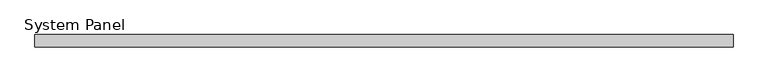
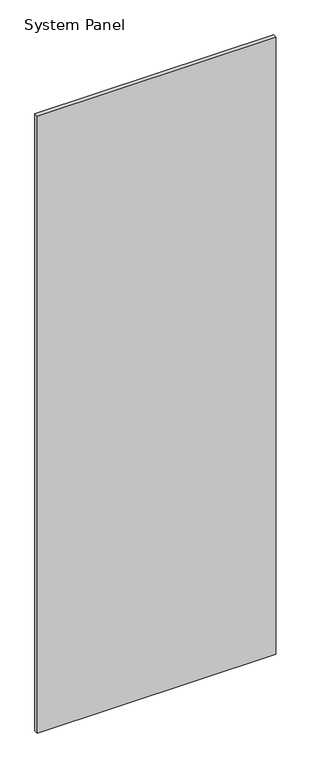
"""IFC4 building model written with IfcOpenShell, lengths in millimetres: plate geometry, System Panel : WWm-Glass-20mm-10mmOffset."""

import ifcopenshell
import ifcopenshell.guid

model = None  # the IFC model being written
_history = None  # IfcOwnerHistory: only IFC2X3 demands one
_inside = {}  # id of a spatial element -> (the spatial element, [elements in it])
_under = {}  # id of a project, library or spatial element -> (it, [spatial elements below it])
_declared = {}  # id of a project -> (the project, [libraries it declares])
_typed = {}  # id of a type object -> (the type object, [elements of that type])
_made_of = {}  # id of a material, layer set ... -> (it, [elements and type objects made of it])


def new_model(schema):
    """Start an empty IFC model of exactly this schema.

    Asked for "IFC4X3", IfcOpenShell would pick the latest addendum, in which some entities
    have other attributes; the version numbers below select the first issue.
    IFC2X3 requires an IfcOwnerHistory on every rooted entity: one is made here for all.
    """
    global model, _history
    if schema == "IFC4X3":
        model = ifcopenshell.file(schema_version=(4, 3, 0, 0))
    else:
        model = ifcopenshell.file(schema=schema)
    _inside.clear()
    _under.clear()
    _declared.clear()
    _typed.clear()
    _made_of.clear()
    _history = None
    if model.schema == "IFC2X3":
        org = make("IfcOrganization", Name="unknown")
        user = make(
            "IfcPersonAndOrganization",
            ThePerson=make("IfcPerson", FamilyName="unknown"),
            TheOrganization=org,
        )
        app = make(
            "IfcApplication",
            ApplicationDeveloper=org,
            Version="unknown",
            ApplicationFullName="unknown",
            ApplicationIdentifier="unknown",
        )
        _history = make(
            "IfcOwnerHistory",
            OwningUser=user,
            OwningApplication=app,
            ChangeAction="ADDED",
            CreationDate=0,
        )
    return model


def make(cls, **values):
    """One entity of the class cls with the attributes given. An attribute that is None is left unset."""
    return model.create_entity(
        cls, **{name: value for name, value in values.items() if value is not None}
    )


def rooted(cls, **values):
    """An entity with a GlobalId (a new one), such as an element, a storey or a relation."""
    return make(cls, GlobalId=ifcopenshell.guid.new(), OwnerHistory=_history, **values)


def si_unit(unit_type, name, prefix=None):
    """IfcSIUnit, for example si_unit("LENGTHUNIT", "METRE", prefix="MILLI")."""
    return make("IfcSIUnit", UnitType=unit_type, Prefix=prefix, Name=name)


def assignment(units):
    """IfcUnitAssignment: the units of a project."""
    return None if units is None else make("IfcUnitAssignment", Units=units)


def point(xyz):
    """IfcCartesianPoint."""
    return None if xyz is None else make("IfcCartesianPoint", Coordinates=xyz)


def direction(xyz):
    """IfcDirection."""
    return None if xyz is None else make("IfcDirection", DirectionRatios=xyz)


def frame(location, z_axis=None, x_axis=None):
    """IfcAxis2Placement3D, a coordinate frame: its origin and axes. An axis left out is left unset."""
    return make(
        "IfcAxis2Placement3D",
        Location=point(location),
        Axis=direction(z_axis),
        RefDirection=direction(x_axis),
    )


def origin():
    """The frame at (0, 0, 0) with its axes left unset."""
    return frame((0.0, 0.0, 0.0))


def origin_with_axes():
    """The frame at (0, 0, 0) with the z axis (0, 0, 1) and the x axis (1, 0, 0) written out."""
    return frame((0.0, 0.0, 0.0), z_axis=(0.0, 0.0, 1.0), x_axis=(1.0, 0.0, 0.0))


def place(relative_to, where):
    """IfcLocalPlacement: puts the frame where relative to a parent placement (None: the world)."""
    return make(
        "IfcLocalPlacement", PlacementRelTo=relative_to, RelativePlacement=where
    )


def context(
    kind, dimensions, precision=None, world=None, true_north=None, identifier=None
):
    """IfcGeometricRepresentationContext, for example the 3D "Model" context."""
    return make(
        "IfcGeometricRepresentationContext",
        ContextIdentifier=identifier,
        ContextType=kind,
        CoordinateSpaceDimension=dimensions,
        Precision=precision,
        WorldCoordinateSystem=world,
        TrueNorth=true_north,
    )


def project(units=None, contexts=None):
    """IfcProject with its units and contexts."""
    return rooted(
        "IfcProject",
        Name="project",
        RepresentationContexts=contexts,
        UnitsInContext=assignment(units),
    )


def spatial(cls, under=None, at=None, **own):
    """A site, building, storey or space (cls), placed at a placement, below another one or the project."""
    s = rooted(cls, ObjectPlacement=at, **own)
    if under is not None:
        _under.setdefault(under.id(), (under, []))[1].append(s)
    return s


def polyline(points):
    """IfcPolyline through the points."""
    return make("IfcPolyline", Points=[point(p) for p in points])


def outline(outer, holes=None, kind="AREA"):
    """IfcArbitraryClosedProfileDef: a profile drawn as a closed curve; with holes, ...WithVoids."""
    if holes is None:
        return make("IfcArbitraryClosedProfileDef", ProfileType=kind, OuterCurve=outer)
    return make(
        "IfcArbitraryProfileDefWithVoids",
        ProfileType=kind,
        OuterCurve=outer,
        InnerCurves=holes,
    )


def extrude(swept, where, along, depth):
    """IfcExtrudedAreaSolid: the profile swept, set in the frame where, extruded along a direction by depth."""
    return make(
        "IfcExtrudedAreaSolid",
        SweptArea=swept,
        Position=where,
        ExtrudedDirection=direction(along),
        Depth=depth,
    )


def shape(context_of_items, identifier, shape_type, items):
    """IfcShapeRepresentation: the items that make up one representation, for example the "Body"."""
    return make(
        "IfcShapeRepresentation",
        ContextOfItems=context_of_items,
        RepresentationIdentifier=identifier,
        RepresentationType=shape_type,
        Items=items,
    )


def source(mapping_origin, context_of_items, identifier, shape_type, items):
    """IfcRepresentationMap: a shape defined once, which mapped items show again and again."""
    return make(
        "IfcRepresentationMap",
        MappingOrigin=mapping_origin,
        MappedRepresentation=shape(context_of_items, identifier, shape_type, items),
    )


def transform(
    local_origin,
    x_axis=None,
    y_axis=None,
    z_axis=None,
    scale=None,
    scale2=None,
    scale3=None,
    uniform=True,
):
    """IfcCartesianTransformationOperator3D, or its non-uniform kind. x_axis, y_axis, z_axis: its Axis1, 2, 3."""
    if uniform:
        return make(
            "IfcCartesianTransformationOperator3D",
            Axis1=direction(x_axis),
            Axis2=direction(y_axis),
            LocalOrigin=point(local_origin),
            Scale=scale,
            Axis3=direction(z_axis),
        )
    return make(
        "IfcCartesianTransformationOperator3DnonUniform",
        Axis1=direction(x_axis),
        Axis2=direction(y_axis),
        LocalOrigin=point(local_origin),
        Scale=scale,
        Axis3=direction(z_axis),
        Scale2=scale2,
        Scale3=scale3,
    )


def mapped(mapping_source, mapping_target):
    """IfcMappedItem: shows the shape of a source again, moved by a transform."""
    return make(
        "IfcMappedItem", MappingSource=mapping_source, MappingTarget=mapping_target
    )


def made_of(thing, what):
    """Note that an element or type object is made of a material, layer set ...; save() writes the relation."""
    if what is not None:
        _made_of.setdefault(what.id(), (what, []))[1].append(thing)
    return thing


def element(
    cls,
    number,
    at=None,
    inside=None,
    cuts=None,
    type_object=None,
    material=None,
    context=None,
    identifier="Body",
    shape_type=None,
    held_by="IfcProductDefinitionShape",
    body=None,
    shapes=None,
    **own,
):
    """One element of the class cls, such as IfcWall. Its Tag is "e" and its number.

    at: its placement. inside: the storey or other place that contains it. cuts: it is an
    opening in that element (IfcRelVoidsElement). A single representation is given by context,
    identifier, shape_type and body (its items); several are given by shapes. held_by: the class
    of the entity that holds the representations. save() writes the other relations.
    """
    e = rooted(cls, Tag="e%d" % number, ObjectPlacement=at, **own)
    if body is not None:
        shapes = [shape(context, identifier, shape_type, body)]
    if shapes is not None:
        e.Representation = make(held_by, Representations=shapes)
    if inside is not None:
        _inside.setdefault(inside.id(), (inside, []))[1].append(e)
    if cuts is not None:
        rooted(
            "IfcRelVoidsElement", RelatingBuildingElement=cuts, RelatedOpeningElement=e
        )
    if type_object is not None:
        _typed.setdefault(type_object.id(), (type_object, []))[1].append(e)
    return made_of(e, material)


def aggregate(whole, parts):
    """IfcRelAggregates: a whole, such as a stair, and the parts it consists of."""
    return rooted("IfcRelAggregates", RelatingObject=whole, RelatedObjects=parts)


def save(model, path):
    """Write the relations noted so far, then the file.

    IfcRelAggregates (storeys below a building ...), IfcRelContainedInSpatialStructure (elements
    in a storey), IfcRelDefinesByType, IfcRelAssociatesMaterial and IfcRelDeclares: one each for
    every whole, place, type object, material and project.
    """
    for whole, parts in _under.values():
        aggregate(whole, parts)
    for where, things in _inside.values():
        rooted(
            "IfcRelContainedInSpatialStructure",
            RelatedElements=things,
            RelatingStructure=where,
        )
    for kind, things in _typed.values():
        rooted("IfcRelDefinesByType", RelatedObjects=things, RelatingType=kind)
    for what, things in _made_of.values():
        rooted("IfcRelAssociatesMaterial", RelatedObjects=things, RelatingMaterial=what)
    for by, libraries in _declared.values():
        rooted("IfcRelDeclares", RelatingContext=by, RelatedDefinitions=libraries)
    model.write(path)


def system_panel_dea0983a(model_context):
    return source(origin(), model_context, "Body", "SweptSolid", [
        extrude(outline(polyline([(576.3545059, 0.0), (-576.3545059, 0.0), (-576.3545059, 20.0), (576.3545059, 20.0), (576.3545059, 0.0)])), origin_with_axes(), (0.0, 0.0, 1.0), 3150.0),
    ])


if __name__ == "__main__":
    model = new_model("IFC4")
    model_context = context("Model", 3, world=origin())
    ifc_project = project(units=[si_unit("LENGTHUNIT", "METRE", prefix="MILLI")], contexts=[model_context])
    site = spatial("IfcSite", under=ifc_project)
    building = spatial("IfcBuilding", under=site)
    placement = place(None, origin())
    system_panel_shape = system_panel_dea0983a(model_context)
    element("IfcPlate", 1, ObjectType="System Panel : WWm-Glass-20mm-10mmOffset", at=placement, inside=building, context=model_context, shape_type="MappedRepresentation", body=[
        mapped(system_panel_shape, transform((0.0, 0.0, 0.0), x_axis=(1.0, 0.0, 0.0), y_axis=(0.0, 1.0, 0.0), z_axis=(0.0, 0.0, 1.0))),
    ])
    save(model, "model.ifc")

# Revit data of these elements
# Type "System Panel : WWm-Glass-20mm-10mmOffset"
#   Finish = ""
# Element 1 (IfcPlate, "System Panel : WWm-Glass-20mm-10mmOffset")
#   Materials on its faces: "WW-EC-GL-Storefront"
# Materials
#   "WW-EC-GL-Storefront": class "Glass", colour RGB 236 240 239, transparency 0.85, Description = "Storefront Glass", Cost = 0
